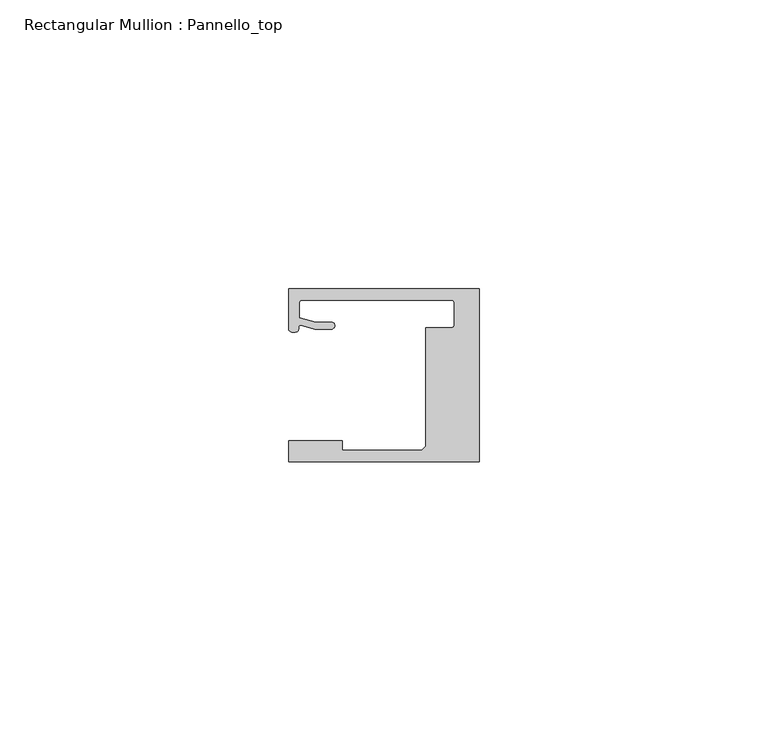
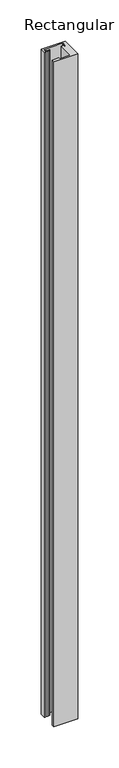
"""IFC4 building model written with IfcOpenShell, lengths in millimetres: member geometry, Rectangular Mullion : Pannello_top."""

from ifc_helpers import new_model, si_unit, frame, origin, place, context, project, spatial, polyline, circle_curve, source, transform, mapped, element, save
from ifc_brep_helpers import plane_surface, cylinder_surface, revolved_surface, extruded_surface, spline_curve, advanced_brep


def rectangular_mullion_pannello_top_98095566(model_context):
    return source(origin(), model_context, "Body", "AdvancedBrep", [
        advanced_brep(
        [(-33.0, -15.0, 0.0), (0.0, -15.0, 0.0), (0.0, 15.0, 0.0), (-33.0000135, 15.0, 0.0), (-33.0000135, 8.0000472, 0.0), (-30.9223017, 8.6490241, 0.0), (-28.4999305, 7.9999523, 0.0), (-25.59998, 7.9999523, 0.0), (-25.59998, 9.1999523, 0.0), (-28.3419477, 9.1999523, 0.0), (-31.19998, 9.9657591, 0.0), (-31.19998, 12.50001, 0.0), (-30.69998, 13.00001, 0.0), (-4.7999726, 13.00001, 0.0), (-4.2999726, 12.50001, 0.0), (-4.2999726, 8.7500595, 0.0), (-4.7999726, 8.2500595, 0.0), (-9.2999726, 8.2500595, 0.0), (-9.2999726, -12.2999849, 0.0), (-10.0000103, -13.0000004, 0.0), (-23.700041, -13.0000004, 0.0), (-23.700041, -11.3000004, 0.0), (-33.0, -11.3000004, 0.0), (-33.0, -15.0, -980.0), (-33.0, -11.3000004, -980.0), (-23.700041, -11.3000004, -980.0), (-23.700041, -13.0000004, -980.0), (-10.0000103, -13.0000004, -980.0), (-9.2999726, -12.2999849, -980.0), (-9.2999726, 8.2500595, -980.0), (-4.7999726, 8.2500595, -980.0), (-4.2999726, 8.7500595, -980.0), (-4.2999726, 12.50001, -980.0), (-4.7999726, 13.00001, -980.0), (-30.69998, 13.00001, -980.0), (-31.19998, 12.50001, -980.0), (-31.19998, 9.9657591, -980.0), (-28.3419477, 9.1999523, -980.0), (-25.59998, 9.1999523, -980.0), (-25.59998, 7.9999523, -980.0), (-28.4999305, 7.9999523, -980.0), (-30.9223017, 8.6490241, -980.0), (-33.0000135, 8.0000472, -980.0), (-33.0000135, 15.0, -980.0), (0.0, 15.0, -980.0), (0.0, -15.0, -980.0)],
        [
            (0, 1),
            (1, 2),
            (2, 3),
            (3, 4),
            (4, 5, spline_curve(3, [(-33.0000135, 8.0000472, 0.0), (-33.0000135, 7.457047519, 0.0), (-32.262327879, 7.456527435, 0.0), (-31.357433266, 7.563996614, 0.0), (-31.305645054, 7.690065204, 0.0), (-31.298563602, 8.366228555, 0.0), (-31.312054066, 8.717747958, 0.0), (-30.9223017, 8.6490241, 0.0)], [4, 2, 2, 4], [0.0, 0.0027053965905959043, 0.0058611956533709, 0.007702013405570312])),
            (5, 6),
            (6, 7),
            (7, 8, circle_curve(frame((-25.59998, 8.5999523, 0.0), z_axis=(0.0, 0.0, 1.0), x_axis=(0.0, 1.0, 0.0)), 0.6)),
            (8, 9),
            (9, 10),
            (10, 11),
            (11, 12, circle_curve(frame((-30.69998, 12.50001, 0.0), z_axis=(0.0, 0.0, -1.0), x_axis=(0.0, 1.0, 0.0)), 0.5)),
            (12, 13),
            (13, 14, circle_curve(frame((-4.7999726, 12.50001, 0.0), z_axis=(0.0, 0.0, -1.0), x_axis=(1.0, 0.0, 0.0)), 0.5)),
            (14, 15),
            (15, 16, circle_curve(frame((-4.7999726, 8.7500595, 0.0), z_axis=(0.0, 0.0, -1.0), x_axis=(0.0, -1.0, 0.0)), 0.5)),
            (16, 17),
            (17, 18),
            (18, 19),
            (19, 20),
            (20, 21),
            (21, 22),
            (22, 0),
            (23, 24),
            (24, 25),
            (25, 26),
            (26, 27),
            (27, 28),
            (28, 29),
            (29, 30),
            (30, 31, circle_curve(frame((-4.7999726, 8.7500595, -980.0), z_axis=(0.0, 0.0, 1.0), x_axis=(0.0, -1.0, 0.0)), 0.5)),
            (31, 32),
            (32, 33, circle_curve(frame((-4.7999726, 12.50001, -980.0), z_axis=(0.0, 0.0, 1.0), x_axis=(1.0, 0.0, 0.0)), 0.5)),
            (33, 34),
            (34, 35, circle_curve(frame((-30.69998, 12.50001, -980.0), z_axis=(0.0, 0.0, 1.0), x_axis=(0.0, 1.0, 0.0)), 0.5)),
            (35, 36),
            (36, 37),
            (37, 38),
            (38, 39, circle_curve(frame((-25.59998, 8.5999523, -980.0), z_axis=(0.0, 0.0, -1.0), x_axis=(0.0, 1.0, 0.0)), 0.6)),
            (39, 40),
            (40, 41),
            (41, 42, spline_curve(3, [(-30.9223017, 8.6490241, -980.0), (-31.312054066, 8.717747958, -980.0), (-31.298563602, 8.366228555, -980.0), (-31.305645054, 7.690065204, -980.0), (-31.357433266, 7.563996614, -980.0), (-32.262327879, 7.456527435, -980.0), (-33.0000135, 7.457047519, -980.0), (-33.0000135, 8.0000472, -980.0)], [4, 2, 2, 4], [0.0, 0.001840817752199412, 0.004996616814974408, 0.007702013405570312])),
            (42, 43),
            (43, 44),
            (44, 45),
            (45, 23),
            (0, 23),
            (45, 1),
            (44, 2),
            (43, 3),
            (42, 4),
            (41, 5),
            (40, 6),
            (39, 7),
            (38, 8),
            (37, 9),
            (36, 10),
            (35, 11),
            (34, 12),
            (33, 13),
            (32, 14),
            (31, 15),
            (30, 16),
            (29, 17),
            (28, 18),
            (27, 19),
            (26, 20),
            (25, 21),
            (24, 22),
        ],
        [
            plane_surface(frame((0.0, -36.2491502, 0.0), z_axis=(0.0, 0.0, 1.0), x_axis=(-1.0, 0.0, 0.0))),
            plane_surface(frame((0.0, -36.2491502, -980.0), z_axis=(0.0, 0.0, -1.0), x_axis=(-1.0, 0.0, 0.0))),
            plane_surface(frame((-33.0, -15.0, 0.0), z_axis=(0.0, -1.0, 0.0), x_axis=(0.0, 0.0, -1.0))),
            plane_surface(frame((0.0, -15.0, 0.0), z_axis=(1.0, 0.0, 0.0), x_axis=(0.0, 0.0, -1.0))),
            plane_surface(frame((0.0, 15.0, 0.0), z_axis=(0.0, 1.0, 0.0), x_axis=(0.0, 0.0, -1.0))),
            plane_surface(frame((-33.0000135, 15.0, 0.0), z_axis=(-1.0, 0.0, 0.0), x_axis=(0.0, 0.0, -1.0))),
            extruded_surface(spline_curve(3, [(-33.0000135, 8.0000472, -980.0), (-33.0000135, 7.457047519, -980.0), (-32.262327879, 7.456527435, -980.0), (-31.357433266, 7.563996614, -980.0), (-31.305645054, 7.690065204, -980.0), (-31.298563602, 8.366228555, -980.0), (-31.312054066, 8.717747958, -980.0), (-30.9223017, 8.6490241, -980.0)], [4, 2, 2, 4], [0.0, 0.0027053965905959043, 0.0058611956533709, 0.007702013405570312]), (0.0, 0.0, 980.0), 980.0),
            plane_surface(frame((-30.9223017, 8.6490241, 0.0), z_axis=(-0.25881883200192934, -0.9659258833891746, 0.0), x_axis=(0.0, 0.0, -1.0))),
            plane_surface(frame((-28.4999305, 7.9999523, 0.0), z_axis=(0.0, -1.0, 0.0), x_axis=(0.0, 0.0, -1.0))),
            cylinder_surface(frame((-25.59998, 8.5999523, 0.0), z_axis=(0.0, 0.0, 1.0), x_axis=(0.0, 1.0, 0.0)), 0.6),
            plane_surface(frame((-25.59998, 9.1999523, 0.0), z_axis=(0.0, 1.0, 0.0), x_axis=(0.0, 0.0, -1.0))),
            plane_surface(frame((-28.3419477, 9.1999523, 0.0), z_axis=(0.25881883204288636, 0.9659258833782002, 0.0), x_axis=(0.0, 0.0, -1.0))),
            plane_surface(frame((-31.19998, 9.9657591, 0.0), z_axis=(1.0, 0.0, 0.0), x_axis=(0.0, 0.0, -1.0))),
            revolved_surface(polyline([(-30.69998, 13.00001, -980.0), (-30.69998, 13.00001, 0.0)]), (-30.69998, 12.50001, 0.0), (0.0, 0.0, -1.0)),
            plane_surface(frame((-30.69998, 13.00001, 0.0), z_axis=(0.0, -1.0, 0.0), x_axis=(0.0, 0.0, -1.0))),
            revolved_surface(polyline([(-4.2999726, 12.50001, -980.0), (-4.2999726, 12.50001, 0.0)]), (-4.7999726, 12.50001, 0.0), (0.0, 0.0, -1.0)),
            plane_surface(frame((-4.2999726, 12.50001, 0.0), z_axis=(-1.0, 0.0, 0.0), x_axis=(0.0, 0.0, -1.0))),
            revolved_surface(polyline([(-4.7999726, 8.2500595, -980.0), (-4.7999726, 8.2500595, 0.0)]), (-4.7999726, 8.7500595, 0.0), (0.0, 0.0, -1.0)),
            plane_surface(frame((-4.7999726, 8.2500595, 0.0), z_axis=(0.0, 1.0, 0.0), x_axis=(0.0, 0.0, -1.0))),
            plane_surface(frame((-9.2999726, 8.2500595, 0.0), z_axis=(-1.0, 0.0, 0.0), x_axis=(0.0, 0.0, -1.0))),
            plane_surface(frame((-9.2999726, -12.2999849, 0.0), z_axis=(-0.7070955486277984, 0.7071180135668678, 0.0), x_axis=(0.0, 0.0, -1.0))),
            plane_surface(frame((-10.0000103, -13.0000004, 0.0), z_axis=(0.0, 1.0, 0.0), x_axis=(0.0, 0.0, -1.0))),
            plane_surface(frame((-23.700041, -13.0000004, 0.0), z_axis=(1.0, 0.0, 0.0), x_axis=(0.0, 0.0, -1.0))),
            plane_surface(frame((-23.700041, -11.3000004, 0.0), z_axis=(0.0, 1.0, 0.0), x_axis=(0.0, 0.0, -1.0))),
            plane_surface(frame((-33.0, -11.3000004, 0.0), z_axis=(-1.0, 0.0, 0.0), x_axis=(0.0, 0.0, -1.0))),
        ],
        [
            (0, [[1, 2, 3, 4, 5, 6, 7, 8, 9, 10, 11, 12, 13, 14, 15, 16, 17, 18, 19, 20, 21, 22, 23]]),
            (1, [[24, 25, 26, 27, 28, 29, 30, 31, 32, 33, 34, 35, 36, 37, 38, 39, 40, 41, 42, 43, 44, 45, 46]]),
            (2, [[-1, 47, -46, 48]]),
            (3, [[-2, -48, -45, 49]]),
            (4, [[-3, -49, -44, 50]]),
            (5, [[-4, -50, -43, 51]]),
            (6, [[-5, -51, -42, 52]]),
            (7, [[-6, -52, -41, 53]]),
            (8, [[-7, -53, -40, 54]]),
            (9, [[-8, -54, -39, 55]]),
            (10, [[-9, -55, -38, 56]]),
            (11, [[-10, -56, -37, 57]]),
            (12, [[-11, -57, -36, 58]]),
            (13, [[-12, -58, -35, 59]]),
            (14, [[-13, -59, -34, 60]]),
            (15, [[-14, -60, -33, 61]]),
            (16, [[-15, -61, -32, 62]]),
            (17, [[-16, -62, -31, 63]]),
            (18, [[-17, -63, -30, 64]]),
            (19, [[-18, -64, -29, 65]]),
            (20, [[-19, -65, -28, 66]]),
            (21, [[-20, -66, -27, 67]]),
            (22, [[-21, -67, -26, 68]]),
            (23, [[-22, -68, -25, 69]]),
            (24, [[-23, -69, -24, -47]]),
        ],
    ),
    ])


if __name__ == "__main__":
    model = new_model("IFC4")
    model_context = context("Model", 3, world=origin())
    ifc_project = project(units=[si_unit("LENGTHUNIT", "METRE", prefix="MILLI")], contexts=[model_context])
    site = spatial("IfcSite", under=ifc_project)
    building = spatial("IfcBuilding", under=site)
    placement = place(None, origin())
    rectangular_mullion_pannello_top_shape = rectangular_mullion_pannello_top_98095566(model_context)
    element("IfcMember", 1, ObjectType="Rectangular Mullion : Pannello_top", at=placement, inside=building, context=model_context, shape_type="MappedRepresentation", body=[
        mapped(rectangular_mullion_pannello_top_shape, transform((0.0, 0.0, 0.0), x_axis=(1.0, 0.0, 0.0), y_axis=(0.0, 1.0, 0.0), z_axis=(0.0, 0.0, 1.0))),
    ])
    save(model, "model.ifc")

# Revit data of these elements
# Type "Rectangular Mullion : Pannello_top"
#   built-in parameter 1007322 = 0.0984252 (stored number, unit not read)
#   built-in parameter 1007321 = 0 (stored number, unit not read)
#   built-in parameter 1007320 = 0.0305117 (stored number, unit not read)
